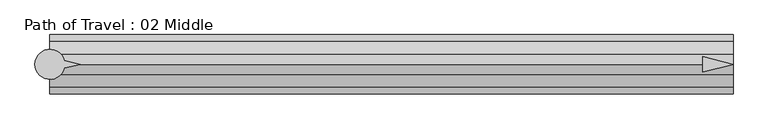
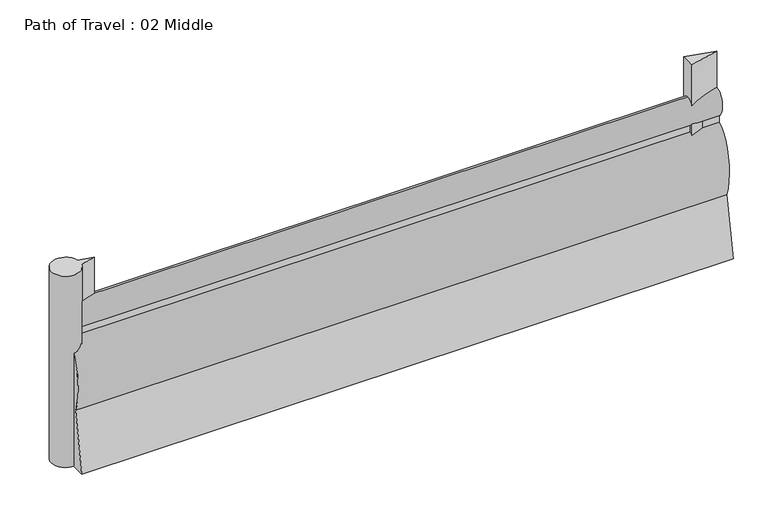
"""IFC4 building model written with IfcOpenShell, lengths in millimetres: proxy geometry, Path of Travel : 02 Middle."""

from ifc_helpers import new_model, si_unit, point, frame, frame_2d, origin, origin_with_axes, place, context, project, spatial, polyline, circle_curve, ellipse_curve, trimmed, segment, composite_curve, outline, extrude, source, transform, mapped, element, save
from ifc_brep_helpers import plane_surface, extruded_surface, advanced_brep


def path_of_travel_02_middle_90690181(model_context):
    return source(origin(), model_context, "Body", "SolidModel", [
        advanced_brep(
        [(227.5554837, 0.0, 1727.2), (227.5554837, 42.9018657, 1436.6534209), (227.5554837, 42.9018657, 1363.4763406), (227.5554837, 184.1186263, 643.4144547), (227.5554837, 297.5699544, 0.0), (227.5554837, 145.6574193, 0.0), (227.5554837, 0.0, 584.2), (227.5554837, -145.6574193, 0.0), (227.5554837, -297.5699544, 0.0), (227.5554837, -184.1186263, 643.4144547), (227.5554837, -42.9018657, 1363.4763406), (227.5554837, -42.9018657, 1436.6534209), (7083.0870372, 0.0, 1727.2), (7083.0870372, -42.9018657, 1436.6534209), (7083.0870372, -42.9018657, 1363.4763406), (7083.0870372, -184.1186263, 643.4144547), (7083.0870372, -297.5699544, 0.0), (7083.0870372, -145.6574193, 0.0), (7083.0870372, 0.0, 584.2), (7083.0870372, 145.6574193, 0.0), (7083.0870372, 297.5699544, 0.0), (7083.0870372, 184.1186263, 643.4144547), (7083.0870372, 42.9018657, 1363.4763406), (7083.0870372, 42.9018657, 1436.6534209)],
        [
            (0, 1, ellipse_curve(frame((227.5554837, 0.0, 1574.8), z_axis=(-1.0, 0.0, 0.0), x_axis=(0.0, 0.0, 1.0)), 152.4, 101.6)),
            (1, 2),
            (2, 3, ellipse_curve(frame((227.5554837, 0.0, 914.4), z_axis=(-1.0, 0.0, 0.0), x_axis=(0.0, 0.0, -1.0)), 457.2, 228.6)),
            (3, 4),
            (4, 5),
            (5, 6),
            (6, 7),
            (7, 8),
            (8, 9),
            (9, 10, ellipse_curve(frame((227.5554837, 0.0, 914.4), z_axis=(-1.0, 0.0, 0.0), x_axis=(0.0, 0.0, -1.0)), 457.2, 228.6)),
            (10, 11),
            (11, 0, ellipse_curve(frame((227.5554837, 0.0, 1574.8), z_axis=(-1.0, 0.0, 0.0), x_axis=(0.0, 0.0, 1.0)), 152.4, 101.6)),
            (12, 13, ellipse_curve(frame((7083.0870372, 0.0, 1574.8), z_axis=(1.0, 0.0, 0.0), x_axis=(0.0, 0.0, 1.0)), 152.4, 101.6)),
            (13, 14),
            (14, 15, ellipse_curve(frame((7083.0870372, 0.0, 914.4), z_axis=(1.0, 0.0, 0.0), x_axis=(0.0, 0.0, -1.0)), 457.2, 228.6)),
            (15, 16),
            (16, 17),
            (17, 18),
            (18, 19),
            (19, 20),
            (20, 21),
            (21, 22, ellipse_curve(frame((7083.0870372, 0.0, 914.4), z_axis=(1.0, 0.0, 0.0), x_axis=(0.0, 0.0, -1.0)), 457.2, 228.6)),
            (22, 23),
            (23, 12, ellipse_curve(frame((7083.0870372, 0.0, 1574.8), z_axis=(1.0, 0.0, 0.0), x_axis=(0.0, 0.0, 1.0)), 152.4, 101.6)),
            (0, 12),
            (23, 1),
            (22, 2),
            (21, 3),
            (20, 4),
            (19, 5),
            (18, 6),
            (17, 7),
            (16, 8),
            (15, 9),
            (14, 10),
            (13, 11),
        ],
        [
            plane_surface(frame((227.5554837, 0.0, 0.0), z_axis=(-1.0, 0.0, 0.0), x_axis=(0.0, 0.0, 1.0))),
            plane_surface(frame((7083.0870372, 0.0, 0.0), z_axis=(1.0, 0.0, 0.0), x_axis=(0.0, 0.0, 1.0))),
            extruded_surface(trimmed(ellipse_curve(frame((7083.0870372, 0.0, 1574.8), z_axis=(-1.0, 0.0, 0.0), x_axis=(0.0, 0.0, 1.0)), 152.4, 101.6), [point((7083.0870372, 0.0, 1727.2))], [point((7083.0870372, 42.9018657, 1436.6534209))], True, "CARTESIAN"), (-6855.5315535, 0.0, 0.0), 6855.5315535),
            plane_surface(frame((227.5554837, 42.9018657, 1436.6534209), z_axis=(0.0, 1.0, 0.0), x_axis=(1.0, 0.0, 0.0))),
            extruded_surface(trimmed(ellipse_curve(frame((7083.0870372, 0.0, 914.4), z_axis=(-1.0, 0.0, 0.0), x_axis=(0.0, 0.0, -1.0)), 457.2, 228.6), [point((7083.0870372, 42.9018657, 1363.4763406))], [point((7083.0870372, 184.1186263, 643.4144547))], True, "CARTESIAN"), (-6855.5315535, 0.0, 0.0), 6855.5315535),
            plane_surface(frame((227.5554837, 184.1186263, 643.4144547), z_axis=(0.0, 0.9848077530122078, 0.1736481776669322), x_axis=(1.0, 0.0, 0.0))),
            plane_surface(frame((227.5554837, 297.5699544, 0.0), z_axis=(0.0, 0.0, -1.0), x_axis=(1.0, 0.0, 0.0))),
            plane_surface(frame((227.5554837, 145.6574193, 0.0), z_axis=(0.0, -0.9702957262760199, -0.2419218955995739), x_axis=(1.0, 0.0, 0.0))),
            plane_surface(frame((227.5554837, 0.0, 584.2), z_axis=(0.0, 0.9702957262759961, -0.24192189559966923), x_axis=(1.0, 0.0, 0.0))),
            plane_surface(frame((227.5554837, -145.6574193, 0.0), z_axis=(0.0, 0.0, -1.0), x_axis=(1.0, 0.0, 0.0))),
            plane_surface(frame((227.5554837, -297.5699544, 0.0), z_axis=(0.0, -0.984807753012208, 0.17364817766693066), x_axis=(1.0, 0.0, 0.0))),
            extruded_surface(trimmed(ellipse_curve(frame((7083.0870372, 0.0, 914.4), z_axis=(-1.0, 0.0, 0.0), x_axis=(0.0, 0.0, -1.0)), 457.2, 228.6), [point((7083.0870372, -184.1186263, 643.4144547))], [point((7083.0870372, -42.9018657, 1363.4763406))], True, "CARTESIAN"), (-6855.5315535, 0.0, 0.0), 6855.5315535),
            plane_surface(frame((227.5554837, -42.9018657, 1363.4763406), z_axis=(0.0, -1.0, 0.0), x_axis=(1.0, 0.0, 0.0))),
            extruded_surface(trimmed(ellipse_curve(frame((7083.0870372, 0.0, 1574.8), z_axis=(-1.0, 0.0, 0.0), x_axis=(0.0, 0.0, 1.0)), 152.4, 101.6), [point((7083.0870372, -42.9018657, 1436.6534209))], [point((7083.0870372, 0.0, 1727.2))], True, "CARTESIAN"), (-6855.5315535, 0.0, 0.0), 6855.5315535),
        ],
        [
            (0, [[1, 2, 3, 4, 5, 6, 7, 8, 9, 10, 11, 12]]),
            (1, [[13, 14, 15, 16, 17, 18, 19, 20, 21, 22, 23, 24]]),
            (2, [[-1, 25, -24, 26]]),
            (3, [[-2, -26, -23, 27]]),
            (4, [[-3, -27, -22, 28]]),
            (5, [[-4, -28, -21, 29]]),
            (6, [[-5, -29, -20, 30]]),
            (7, [[-6, -30, -19, 31]]),
            (8, [[-7, -31, -18, 32]]),
            (9, [[-8, -32, -17, 33]]),
            (10, [[-9, -33, -16, 34]]),
            (11, [[-10, -34, -15, 35]]),
            (12, [[-11, -35, -14, 36]]),
            (13, [[-12, -36, -13, -25]]),
        ],
    ),
        extrude(outline(polyline([(6777.0818907, 76.2006338), (7083.0870372, 0.0), (6777.0818907, -76.2006338), (6777.0818907, 76.2006338)])), origin_with_axes(), (0.0, 0.0, 1.0), 2129.5973753),
        extrude(outline(composite_curve([segment(polyline([(372.7837828, 39.4440225), (531.182385, 0.0), (372.7837828, -39.4440225)]), True, "CONTINUOUS"), segment(trimmed(circle_curve(frame_2d((227.2200886, 0.0)), 150.8131956), [point((372.7837828, -39.4440225))], [point((372.7837828, 39.4440225))], False, "CARTESIAN"), True, "CONTINUOUS")], self_intersect=False)), origin_with_axes(), (0.0, 0.0, 1.0), 2129.5973753),
    ])


if __name__ == "__main__":
    model = new_model("IFC4")
    model_context = context("Model", 3, world=origin())
    ifc_project = project(units=[si_unit("LENGTHUNIT", "METRE", prefix="MILLI")], contexts=[model_context])
    site = spatial("IfcSite", under=ifc_project)
    building = spatial("IfcBuilding", under=site)
    placement = place(None, origin())
    path_of_travel_02_middle_shape = path_of_travel_02_middle_90690181(model_context)
    element("IfcBuildingElementProxy", 1, Name="Path of Travel : 02 Middle", ObjectType="Path of Travel : 02 Middle", at=placement, inside=building, context=model_context, shape_type="MappedRepresentation", body=[
        mapped(path_of_travel_02_middle_shape, transform((0.0, 0.0, 0.0), x_axis=(1.0, 0.0, 0.0), y_axis=(0.0, 1.0, 0.0), z_axis=(0.0, 0.0, 1.0))),
    ])
    save(model, "model.ifc")

# Revit data of these elements
# Type "Path of Travel : 02 Middle"
#   Path of Egress [instance default] = 4' - 0"
#   built-in parameter 1001306 [instance default] = 4 (stored number, unit not read)
#   Dot at Start = no
#   Arrow in Middle = yes
#   Arrow at End = no
#   Egress Path = none
# Element 1 (IfcBuildingElementProxy, "Path of Travel : 02 Middle")
#   Path of Egress = 22' - 5.90282"
#   built-in parameter 1001306 = 22.4919 (stored number, unit not read)
#   Materials on its faces: "Egress Path Solid", "solid"
# Materials
#   "Egress Path Solid": class "Unassigned", colour RGB 255 128 64, transparency 0.75, Comments = "Rendering appearance not upgraded "
#   "solid": class "Generic", colour RGB 120 120 120, transparency 0, Cost = 0
